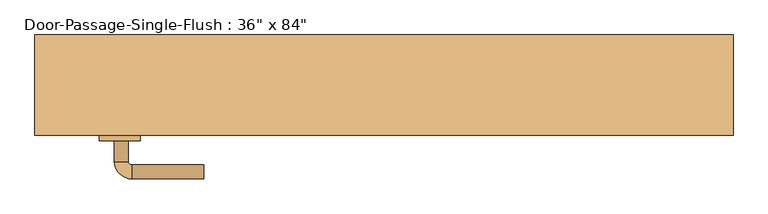
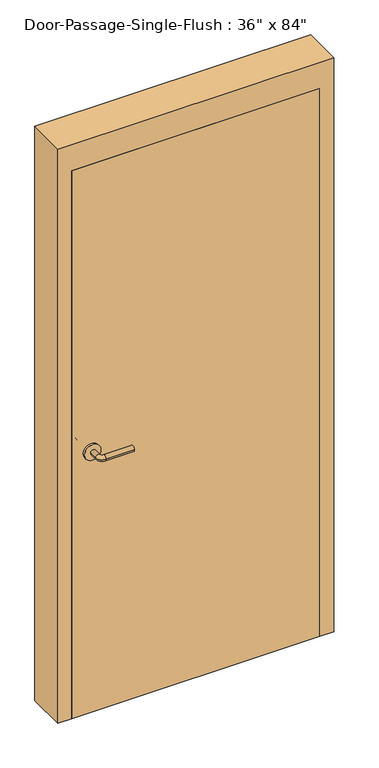
"""IFC4 building model written with IfcOpenShell, lengths in millimetres: door geometry."""

from ifc_helpers import new_model, si_unit, point, frame, frame_2d, origin, origin_with_axes, place, context, project, spatial, polyline, circle_curve, ellipse_curve, trimmed, segment, composite_curve, outline, extrude, faceted_brep, source, transform, mapped, element, save
from ifc_brep_helpers import plane_surface, cylinder_surface, revolved_surface, advanced_brep


def door_2b15ddfc(model_context):
    return source(origin(), model_context, "Body", "SolidModel", [
        advanced_brep(
        [(-392.190625, -155.5125, 1016.0), (-372.190625, -155.5125, 1016.0), (-392.190625, -125.5125, 1016.0), (-372.190625, -125.5125, 1016.0), (-367.190625, -120.5125, 1016.0), (-367.190625, -100.5125, 1016.0), (-262.190625, -100.5125, 1016.0), (-262.190625, -120.5125, 1016.0)],
        [
            (0, 1, circle_curve(frame((-382.190625, -155.5125, 1016.0), z_axis=(0.0, -1.0, 0.0), x_axis=(1.0, 0.0, 0.0)), 10.0)),
            (1, 0, circle_curve(frame((-382.190625, -155.5125, 1016.0), z_axis=(0.0, -1.0, 0.0), x_axis=(1.0, 0.0, 0.0)), 10.0)),
            (0, 2),
            (2, 3, circle_curve(frame((-382.190625, -125.5125, 1016.0), z_axis=(0.0, -1.0, 0.0), x_axis=(1.0, 0.0, 0.0)), 10.0)),
            (3, 1),
            (3, 2, circle_curve(frame((-382.190625, -125.5125, 1016.0), z_axis=(0.0, -1.0, 0.0), x_axis=(1.0, 0.0, 0.0)), 10.0)),
            (4, 3, circle_curve(frame((-367.190625, -125.5125, 1016.0), z_axis=(0.0, 0.0, 1.0), x_axis=(-1.0, 0.0, 0.0)), 5.0)),
            (2, 5, circle_curve(frame((-367.190625, -125.5125, 1016.0), z_axis=(0.0, 0.0, -1.0), x_axis=(-1.0, 0.0, 0.0)), 25.0)),
            (5, 4, circle_curve(frame((-367.190625, -110.5125, 1016.0), z_axis=(-1.0, 0.0, 0.0), x_axis=(0.0, -1.0, 0.0)), 10.0)),
            (4, 5, circle_curve(frame((-367.190625, -110.5125, 1016.0), z_axis=(-1.0, 0.0, 0.0), x_axis=(0.0, -1.0, 0.0)), 10.0)),
            (6, 7, circle_curve(frame((-262.190625, -110.5125, 1016.0), z_axis=(1.0, 0.0, 0.0), x_axis=(0.0, -1.0, 0.0)), 10.0)),
            (7, 6, circle_curve(frame((-262.190625, -110.5125, 1016.0), z_axis=(1.0, 0.0, 0.0), x_axis=(0.0, -1.0, 0.0)), 10.0)),
            (5, 6),
            (7, 4),
        ],
        [
            plane_surface(frame((-382.190625, -155.5125, 1016.0), z_axis=(0.0, -1.0, 0.0), x_axis=(0.0, 0.0, 1.0))),
            cylinder_surface(frame((-382.190625, -155.5125, 1016.0), z_axis=(0.0, -1.0, 0.0), x_axis=(1.0, 0.0, 0.0)), 10.0),
            revolved_surface(trimmed(ellipse_curve(frame((-382.190625, -125.5125, 1016.0), z_axis=(0.0, -1.0, 0.0), x_axis=(1.0, 0.0, 0.0)), 10.0, 10.0), [point((-392.190625, -125.5125, 1016.0))], [point((-372.190625, -125.5125, 1016.0))], True, "CARTESIAN"), (-367.190625, -125.5125, 1016.0), (0.0, 0.0, -1.0)),
            revolved_surface(trimmed(ellipse_curve(frame((-382.190625, -125.5125, 1016.0), z_axis=(0.0, -1.0, 0.0), x_axis=(1.0, 0.0, 0.0)), 10.0, 10.0), [point((-372.190625, -125.5125, 1016.0))], [point((-392.190625, -125.5125, 1016.0))], True, "CARTESIAN"), (-367.190625, -125.5125, 1016.0), (0.0, 0.0, -1.0)),
            plane_surface(frame((-262.190625, -110.5125, 1016.0), z_axis=(1.0, 0.0, 0.0), x_axis=(0.0, 0.0, 1.0))),
            cylinder_surface(frame((-367.190625, -110.5125, 1016.0), z_axis=(-1.0, 0.0, 0.0), x_axis=(0.0, -1.0, 0.0)), 10.0),
        ],
        [
            (0, [[1, 2]]),
            (1, [[-1, 3, 4, 5]]),
            (1, [[-2, -5, 6, -3]]),
            (2, [[7, -4, 8, 9]]),
            (3, [[-8, -6, -7, 10]]),
            (4, [[11, 12]]),
            (5, [[-9, 13, -12, 14]]),
            (5, [[-10, -14, -11, -13]]),
        ],
    ),
        extrude(outline(composite_curve([segment(trimmed(circle_curve(frame_2d((1016.0, -384.690625)), 30.0), [point((1016.0, -414.690625))], [point((1016.0, -354.690625))], False, "CARTESIAN"), True, "CONTINUOUS"), segment(trimmed(circle_curve(frame_2d((1016.0, -384.690625)), 30.0), [point((1016.0, -354.690625))], [point((1016.0, -414.690625))], False, "CARTESIAN"), True, "CONTINUOUS")], self_intersect=False)), frame((0.0, -163.5125, 0.0), z_axis=(0.0, 1.0, 0.0), x_axis=(0.0, 0.0, 1.0)), (0.0, 0.0, 1.0), 8.0),
        advanced_brep(
        [(-392.190625, -215.9625, 1016.0), (-372.190625, -215.9625, 1016.0), (-372.190625, -245.9625, 1016.0), (-392.190625, -245.9625, 1016.0), (-367.190625, -250.9625, 1016.0), (-367.190625, -270.9625, 1016.0), (-262.190625, -270.9625, 1016.0), (-262.190625, -250.9625, 1016.0)],
        [
            (0, 1, circle_curve(frame((-382.190625, -215.9625, 1016.0), z_axis=(0.0, 1.0, 0.0), x_axis=(1.0, 0.0, 0.0)), 10.0)),
            (1, 0, circle_curve(frame((-382.190625, -215.9625, 1016.0), z_axis=(0.0, 1.0, 0.0), x_axis=(1.0, 0.0, 0.0)), 10.0)),
            (1, 2),
            (2, 3, circle_curve(frame((-382.190625, -245.9625, 1016.0), z_axis=(0.0, 1.0, 0.0), x_axis=(1.0, 0.0, 0.0)), 10.0)),
            (3, 0),
            (3, 2, circle_curve(frame((-382.190625, -245.9625, 1016.0), z_axis=(0.0, 1.0, 0.0), x_axis=(1.0, 0.0, 0.0)), 10.0)),
            (4, 5, circle_curve(frame((-367.190625, -260.9625, 1016.0), z_axis=(-1.0, 0.0, 0.0), x_axis=(0.0, 1.0, 0.0)), 10.0)),
            (5, 3, circle_curve(frame((-367.190625, -245.9625, 1016.0), z_axis=(0.0, 0.0, -1.0), x_axis=(-1.0, 0.0, 0.0)), 25.0)),
            (2, 4, circle_curve(frame((-367.190625, -245.9625, 1016.0), z_axis=(0.0, 0.0, 1.0), x_axis=(-1.0, 0.0, 0.0)), 5.0)),
            (5, 4, circle_curve(frame((-367.190625, -260.9625, 1016.0), z_axis=(-1.0, 0.0, 0.0), x_axis=(0.0, 1.0, 0.0)), 10.0)),
            (6, 7, circle_curve(frame((-262.190625, -260.9625, 1016.0), z_axis=(1.0, 0.0, 0.0), x_axis=(0.0, 1.0, 0.0)), 10.0)),
            (7, 6, circle_curve(frame((-262.190625, -260.9625, 1016.0), z_axis=(1.0, 0.0, 0.0), x_axis=(0.0, 1.0, 0.0)), 10.0)),
            (4, 7),
            (6, 5),
        ],
        [
            plane_surface(frame((-382.190625, -215.9625, 1016.0), z_axis=(0.0, 1.0, 0.0), x_axis=(0.0, 0.0, 1.0))),
            cylinder_surface(frame((-382.190625, -215.9625, 1016.0), z_axis=(0.0, 1.0, 0.0), x_axis=(1.0, 0.0, 0.0)), 10.0),
            revolved_surface(trimmed(ellipse_curve(frame((-382.190625, -245.9625, 1016.0), z_axis=(0.0, -1.0, 0.0), x_axis=(1.0, 0.0, 0.0)), 10.0, 10.0), [point((-392.190625, -245.9625, 1016.0))], [point((-372.190625, -245.9625, 1016.0))], True, "CARTESIAN"), (-367.190625, -245.9625, 1016.0), (0.0, 0.0, -1.0)),
            revolved_surface(trimmed(ellipse_curve(frame((-382.190625, -245.9625, 1016.0), z_axis=(0.0, -1.0, 0.0), x_axis=(1.0, 0.0, 0.0)), 10.0, 10.0), [point((-372.190625, -245.9625, 1016.0))], [point((-392.190625, -245.9625, 1016.0))], True, "CARTESIAN"), (-367.190625, -245.9625, 1016.0), (0.0, 0.0, -1.0)),
            plane_surface(frame((-262.190625, -260.9625, 1016.0), z_axis=(1.0, 0.0, 0.0), x_axis=(0.0, 0.0, 1.0))),
            cylinder_surface(frame((-367.190625, -260.9625, 1016.0), z_axis=(-1.0, 0.0, 0.0), x_axis=(0.0, 1.0, 0.0)), 10.0),
        ],
        [
            (0, [[1, 2]]),
            (1, [[3, 4, 5, -2]]),
            (1, [[-5, 6, -3, -1]]),
            (2, [[7, 8, -4, 9]]),
            (3, [[10, -9, -6, -8]]),
            (4, [[11, 12]]),
            (5, [[13, -11, 14, -7]]),
            (5, [[-14, -12, -13, -10]]),
        ],
    ),
        extrude(outline(composite_curve([segment(trimmed(circle_curve(frame_2d((1016.0, -384.690625)), 30.0), [point((1016.0, -414.690625))], [point((1016.0, -354.690625))], False, "CARTESIAN"), True, "CONTINUOUS"), segment(trimmed(circle_curve(frame_2d((1016.0, -384.690625)), 30.0), [point((1016.0, -354.690625))], [point((1016.0, -414.690625))], False, "CARTESIAN"), True, "CONTINUOUS")], self_intersect=False)), frame((0.0, -215.9625, 0.0), z_axis=(0.0, 1.0, 0.0), x_axis=(0.0, 0.0, 1.0)), (0.0, 0.0, 1.0), 8.0),
        faceted_brep([(457.2, -158.75, 0.0), (441.325, -158.75, 0.0), (441.325, -111.125, 0.0), (457.2, -111.125, 0.0), (457.2, -61.9125, 0.0), (508.0, -61.9125, 0.0), (508.0, -207.9625, 0.0), (457.2, -207.9625, 0.0), (457.2, -207.9625, 2133.6), (457.2, -158.75, 2133.6), (508.0, -207.9625, 2235.2), (-508.0, -207.9625, 2235.2), (-508.0, -207.9625, 0.0), (-457.2, -207.9625, 0.0), (-457.2, -207.9625, 2133.6), (508.0, -61.9125, 2235.2), (457.2, -61.9125, 2133.6), (-457.2, -61.9125, 2133.6), (-457.2, -61.9125, 0.0), (-508.0, -61.9125, 0.0), (-508.0, -61.9125, 2235.2), (457.2, -111.125, 2133.6), (441.325, -111.125, 2117.725), (-441.325, -111.125, 2117.725), (-441.325, -111.125, 0.0), (-457.2, -111.125, 0.0), (-457.2, -111.125, 2133.6), (441.325, -158.75, 2117.725), (-457.2, -158.75, 2133.6), (-457.2, -158.75, 0.0), (-441.325, -158.75, 0.0), (-441.325, -158.75, 2117.725)], [[[0, 1, 2, 3, 4, 5, 6, 7]], [[7, 8, 9, 0]], [[6, 10, 11, 12, 13, 14, 8, 7]], [[5, 15, 10, 6]], [[4, 16, 17, 18, 19, 20, 15, 5]], [[3, 21, 16, 4]], [[2, 22, 23, 24, 25, 26, 21, 3]], [[1, 27, 22, 2]], [[0, 9, 28, 29, 30, 31, 27, 1]], [[8, 14, 28, 9]], [[16, 21, 26, 17]], [[22, 27, 31, 23]], [[12, 19, 18, 25, 24, 30, 29, 13]], [[13, 29, 28, 14]], [[11, 20, 19, 12]], [[17, 26, 25, 18]], [[23, 31, 30, 24]], [[15, 20, 11, 10]]]),
        extrude(outline(polyline([(457.2, -163.5125), (457.2, -207.9625), (-457.2, -207.9625), (-457.2, -163.5125), (457.2, -163.5125)])), origin_with_axes(), (0.0, 0.0, 1.0), 2133.6),
    ])


if __name__ == "__main__":
    model = new_model("IFC4")
    model_context = context("Model", 3, world=origin())
    ifc_project = project(units=[si_unit("LENGTHUNIT", "METRE", prefix="MILLI")], contexts=[model_context])
    site = spatial("IfcSite", under=ifc_project)
    building = spatial("IfcBuilding", under=site)
    placement = place(None, origin())
    door_shape = door_2b15ddfc(model_context)
    element("IfcDoor", 1, ObjectType="Door-Passage-Single-Flush : 36\" x 84\"", at=placement, inside=building, context=model_context, shape_type="MappedRepresentation", body=[
        mapped(door_shape, transform((0.0, 0.0, 0.0), x_axis=(1.0, 0.0, 0.0), y_axis=(0.0, 1.0, 0.0), z_axis=(0.0, 0.0, 1.0))),
    ])
    save(model, "model.ifc")

# Revit data of these elements
# Type "Door-Passage-Single-Flush : 36\" x 84\""
#   Type Mark = "35"
#   Assembly Code = "B2030200"
#   Analytic Construction = "Wooden"
#   Thickness = 0' - 1 3/4"
#   Thermal Resistance (R) = 2.5876 (h·ft²·°F)/BTU
#   Swing Angle [instance default] = 90.00°
#   Strike Height = 3' - 4"
#   Rough Width [instance default] = 3' - 4"
#   Rough Height [instance default] = 7' - 4"
#   MF Opening Height [instance default] = 0' - 4"
#   MF Opening Width [instance default] = 0' - 4"
#   Inset Calculate [instance default] = 0' - 4"
#   Masonry Inset [instance default] = 0' - 1"
#   Height = 7' - 0"
#   Width = 3' - 0"
#   Heat Transfer Coefficient (U) = 0.3865 BTU/(h·ft²·°F)
#   Masonry Frame Depth = 0' - 5 3/4"
#   Masonry Frame [instance default] = yes
#   Function = 1
#   Dry Wall Frame [instance default] = no
#   Panel Material = Wood - Birch
#   Frame Material = Metal - Paint Finish - Grey
#   Door Handle Material = Aluminum
#   Visual Light Transmittance = 0
#   Solar Heat Gain Coefficient = 0
#   Wall Closure = (empty or 0)
# Element 1 (IfcDoor, "Door-Passage-Single-Flush : 36\" x 84\"")
#   Materials on its faces: "Aluminum", "Metal - Paint Finish - Grey", "Wood - Birch"
# Materials
#   "Wood - Birch": class "Wood", colour RGB 166 116 52, transparency 0, Cost = 0
#   "Metal - Paint Finish - Grey": class "Paint", colour RGB 104 104 104, transparency 0, Cost = 0
#   "Aluminum": class "Metal", colour RGB 247 247 247, transparency 0, Description = "Aluminum 6061", Cost = 0
